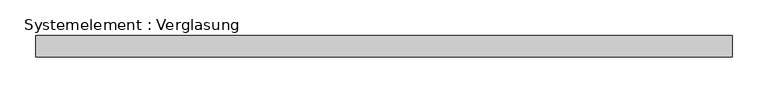
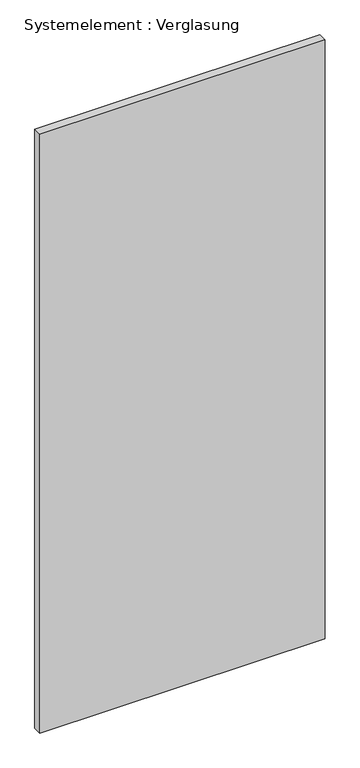
"""IFC4 building model written with IfcOpenShell, lengths in millimetres: plate geometry, Systemelement : Verglasung."""

from ifc_helpers import new_model, si_unit, origin, origin_with_axes, place, context, project, spatial, polyline, outline, extrude, source, transform, mapped, element, save


def systemelement_verglasung_556215b4(model_context):
    return source(origin(), model_context, "Body", "SweptSolid", [
        extrude(outline(polyline([(486.6118989, -15.0), (-486.6118989, -15.0), (-486.6118989, 15.0), (486.6118989, 15.0), (486.6118989, -15.0)])), origin_with_axes(), (0.0, 0.0, 1.0), 2160.0),
    ])


if __name__ == "__main__":
    model = new_model("IFC4")
    model_context = context("Model", 3, world=origin())
    ifc_project = project(units=[si_unit("LENGTHUNIT", "METRE", prefix="MILLI")], contexts=[model_context])
    site = spatial("IfcSite", under=ifc_project)
    building = spatial("IfcBuilding", under=site)
    placement = place(None, origin())
    systemelement_verglasung_shape = systemelement_verglasung_556215b4(model_context)
    element("IfcPlate", 1, ObjectType="Systemelement : Verglasung", at=placement, inside=building, context=model_context, shape_type="MappedRepresentation", body=[
        mapped(systemelement_verglasung_shape, transform((0.0, 0.0, 0.0), x_axis=(1.0, 0.0, 0.0), y_axis=(0.0, 1.0, 0.0), z_axis=(0.0, 0.0, 1.0))),
    ])
    save(model, "model.ifc")

# Revit data of these elements
# Type "Systemelement : Verglasung"
#   Construction Type Id = "GSP4R"
#   Analytic Construction = "1/8 Zoll Pilkington-Verglasung einfach"
#   Visual Light Transmittance = 0.9
#   Solar Heat Gain Coefficient = 0.86
#   Heat Transfer Coefficient (U) = 6.7069 W/(m²·K)
# Element 1 (IfcPlate, "Systemelement : Verglasung")
#   Materials on its faces: "Glas"
# Materials
#   "Glas": class "Glas", colour RGB 0 0 255, transparency 0.75, Comments = "Render-Darstellung nicht aktualisiert ", Cost = 0
